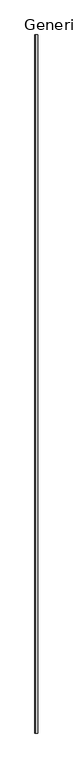
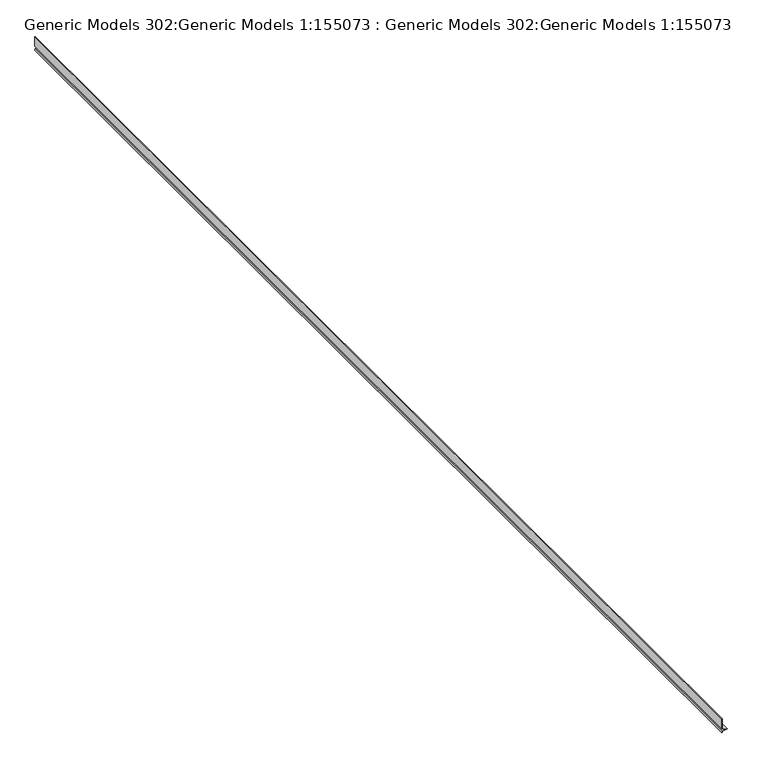
"""IFC4 building model written with IfcOpenShell, lengths in millimetres: proxy geometry, Generic Models 302:Generic Models 1:155073 : Generic Models 302:Generic Models 1:155073."""

from ifc_helpers import new_model, si_unit, frame, origin, place, context, project, spatial, polyline, outline, extrude, source, transform, mapped, element, save


def generic_models_302_generic_models_1_155073_generic_models_5ad12170(model_context):
    return source(origin(), model_context, "Body", "SweptSolid", [
        extrude(outline(polyline([(130.9730521, 6834.5495965), (137.4510003, 6854.703213), (144.186536, 6833.748213), (188.2510003, 6833.748213), (188.2510003, 6832.478213), (143.2607567, 6832.478213), (137.4510003, 6850.5530108), (131.9508423, 6833.4414081), (126.8360919, 6832.478213), (126.6010604, 6833.7262756), (130.9730521, 6834.5495965)])), frame((0.0, 7041.2025207, 0.0), z_axis=(0.0, 1.0, 0.0), x_axis=(0.0, 0.0, 1.0)), (0.0, 0.0, 1.0), 5130.8),
    ])


if __name__ == "__main__":
    model = new_model("IFC4")
    model_context = context("Model", 3, world=origin())
    ifc_project = project(units=[si_unit("LENGTHUNIT", "METRE", prefix="MILLI")], contexts=[model_context])
    site = spatial("IfcSite", under=ifc_project)
    building = spatial("IfcBuilding", under=site)
    placement = place(None, origin())
    generic_models_302_generic_models_1_155073_generic_models_shape = generic_models_302_generic_models_1_155073_generic_models_5ad12170(model_context)
    element("IfcBuildingElementProxy", 1, Name="Generic Models 302:Generic Models 1:155073 : Generic Models 302:Generic Models 1:155073", ObjectType="Generic Models 302:Generic Models 1:155073 : Generic Models 302:Generic Models 1:155073", at=placement, inside=building, context=model_context, shape_type="MappedRepresentation", body=[
        mapped(generic_models_302_generic_models_1_155073_generic_models_shape, transform((0.0, 0.0, 0.0), x_axis=(1.0, 0.0, 0.0), y_axis=(0.0, 1.0, 0.0), z_axis=(0.0, 0.0, 1.0))),
    ])
    save(model, "model.ifc")

# Revit data of these elements
# Type "Generic Models 302:Generic Models 1:155073 : Generic Models 302:Generic Models 1:155073"
#   NameOverride = "Generic Models 302:Generic Models 1:155073"
#   ObjectTypeOverride = "Generic Models 302:Generic Models 1"
#   Reference = "Generic Models 1"
#   Category = "Generic Models"
#   Tag = "155073"
# Element 1 (IfcBuildingElementProxy, "Generic Models 302:Generic Models 1:155073 : Generic Models 302:Generic Models 1:155073")
#   Materials on its faces: "_16 GA. COPPER WEEP SCREED W/ MIN. 3 1/2\" ATTACHEMENT FLANGE - LAP UNDERLAYMENT OVER WEED SCREED 3430"
# Materials
#   "_16 GA. COPPER WEEP SCREED W/ MIN. 3 1/2\" ATTACHEMENT FLANGE - LAP UNDERLAYMENT OVER WEED SCREED 3430": class "Unassigned", colour RGB 253 192 103, transparency 0
